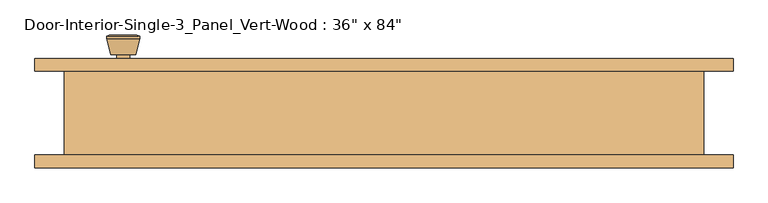
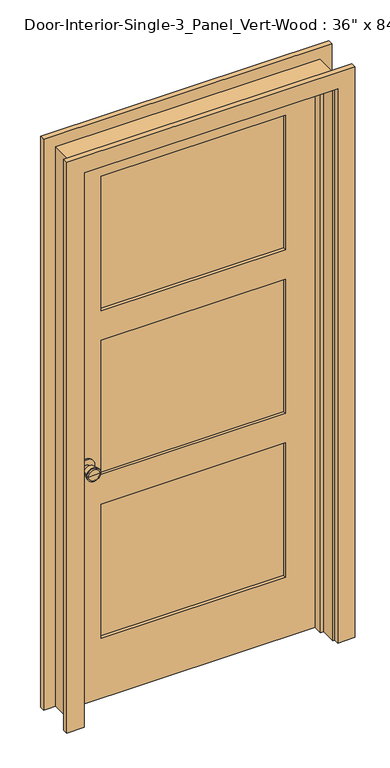
"""IFC4 building model written with IfcOpenShell, lengths in millimetres: door geometry."""

import ifcopenshell
import ifcopenshell.guid

model = None  # the IFC model being written
_history = None  # IfcOwnerHistory: only IFC2X3 demands one
_inside = {}  # id of a spatial element -> (the spatial element, [elements in it])
_under = {}  # id of a project, library or spatial element -> (it, [spatial elements below it])
_declared = {}  # id of a project -> (the project, [libraries it declares])
_typed = {}  # id of a type object -> (the type object, [elements of that type])
_made_of = {}  # id of a material, layer set ... -> (it, [elements and type objects made of it])


def new_model(schema):
    """Start an empty IFC model of exactly this schema.

    Asked for "IFC4X3", IfcOpenShell would pick the latest addendum, in which some entities
    have other attributes; the version numbers below select the first issue.
    IFC2X3 requires an IfcOwnerHistory on every rooted entity: one is made here for all.
    """
    global model, _history
    if schema == "IFC4X3":
        model = ifcopenshell.file(schema_version=(4, 3, 0, 0))
    else:
        model = ifcopenshell.file(schema=schema)
    _inside.clear()
    _under.clear()
    _declared.clear()
    _typed.clear()
    _made_of.clear()
    _history = None
    if model.schema == "IFC2X3":
        org = make("IfcOrganization", Name="unknown")
        user = make(
            "IfcPersonAndOrganization",
            ThePerson=make("IfcPerson", FamilyName="unknown"),
            TheOrganization=org,
        )
        app = make(
            "IfcApplication",
            ApplicationDeveloper=org,
            Version="unknown",
            ApplicationFullName="unknown",
            ApplicationIdentifier="unknown",
        )
        _history = make(
            "IfcOwnerHistory",
            OwningUser=user,
            OwningApplication=app,
            ChangeAction="ADDED",
            CreationDate=0,
        )
    return model


def make(cls, **values):
    """One entity of the class cls with the attributes given. An attribute that is None is left unset."""
    return model.create_entity(
        cls, **{name: value for name, value in values.items() if value is not None}
    )


def rooted(cls, **values):
    """An entity with a GlobalId (a new one), such as an element, a storey or a relation."""
    return make(cls, GlobalId=ifcopenshell.guid.new(), OwnerHistory=_history, **values)


def si_unit(unit_type, name, prefix=None):
    """IfcSIUnit, for example si_unit("LENGTHUNIT", "METRE", prefix="MILLI")."""
    return make("IfcSIUnit", UnitType=unit_type, Prefix=prefix, Name=name)


def assignment(units):
    """IfcUnitAssignment: the units of a project."""
    return None if units is None else make("IfcUnitAssignment", Units=units)


def point(xyz):
    """IfcCartesianPoint."""
    return None if xyz is None else make("IfcCartesianPoint", Coordinates=xyz)


def direction(xyz):
    """IfcDirection."""
    return None if xyz is None else make("IfcDirection", DirectionRatios=xyz)


def frame(location, z_axis=None, x_axis=None):
    """IfcAxis2Placement3D, a coordinate frame: its origin and axes. An axis left out is left unset."""
    return make(
        "IfcAxis2Placement3D",
        Location=point(location),
        Axis=direction(z_axis),
        RefDirection=direction(x_axis),
    )


def frame_2d(location, x_axis=None):
    """IfcAxis2Placement2D, a coordinate frame in the plane: its origin and x axis."""
    return make(
        "IfcAxis2Placement2D", Location=point(location), RefDirection=direction(x_axis)
    )


def origin():
    """The frame at (0, 0, 0) with its axes left unset."""
    return frame((0.0, 0.0, 0.0))


def place(relative_to, where):
    """IfcLocalPlacement: puts the frame where relative to a parent placement (None: the world)."""
    return make(
        "IfcLocalPlacement", PlacementRelTo=relative_to, RelativePlacement=where
    )


def context(
    kind, dimensions, precision=None, world=None, true_north=None, identifier=None
):
    """IfcGeometricRepresentationContext, for example the 3D "Model" context."""
    return make(
        "IfcGeometricRepresentationContext",
        ContextIdentifier=identifier,
        ContextType=kind,
        CoordinateSpaceDimension=dimensions,
        Precision=precision,
        WorldCoordinateSystem=world,
        TrueNorth=true_north,
    )


def project(units=None, contexts=None):
    """IfcProject with its units and contexts."""
    return rooted(
        "IfcProject",
        Name="project",
        RepresentationContexts=contexts,
        UnitsInContext=assignment(units),
    )


def spatial(cls, under=None, at=None, **own):
    """A site, building, storey or space (cls), placed at a placement, below another one or the project."""
    s = rooted(cls, ObjectPlacement=at, **own)
    if under is not None:
        _under.setdefault(under.id(), (under, []))[1].append(s)
    return s


def polyline(points):
    """IfcPolyline through the points."""
    return make("IfcPolyline", Points=[point(p) for p in points])


def circle_curve(where, radius):
    """IfcCircle in the frame where."""
    return make("IfcCircle", Position=where, Radius=radius)


def trimmed(basis, trim1, trim2, sense, master):
    """IfcTrimmedCurve: the piece of a basis curve between two trims."""
    return make(
        "IfcTrimmedCurve",
        BasisCurve=basis,
        Trim1=trim1,
        Trim2=trim2,
        SenseAgreement=sense,
        MasterRepresentation=master,
    )


def segment(curve, same_sense, transition):
    """IfcCompositeCurveSegment."""
    return make(
        "IfcCompositeCurveSegment",
        Transition=transition,
        SameSense=same_sense,
        ParentCurve=curve,
    )


def composite_curve(segments, self_intersect=None):
    """IfcCompositeCurve: segments joined end to end."""
    return make("IfcCompositeCurve", Segments=segments, SelfIntersect=self_intersect)


def outline(outer, holes=None, kind="AREA"):
    """IfcArbitraryClosedProfileDef: a profile drawn as a closed curve; with holes, ...WithVoids."""
    if holes is None:
        return make("IfcArbitraryClosedProfileDef", ProfileType=kind, OuterCurve=outer)
    return make(
        "IfcArbitraryProfileDefWithVoids",
        ProfileType=kind,
        OuterCurve=outer,
        InnerCurves=holes,
    )


def extrude(swept, where, along, depth):
    """IfcExtrudedAreaSolid: the profile swept, set in the frame where, extruded along a direction by depth."""
    return make(
        "IfcExtrudedAreaSolid",
        SweptArea=swept,
        Position=where,
        ExtrudedDirection=direction(along),
        Depth=depth,
    )


def faces_of(points, faces, orient=None, outer=None):
    """IfcFace entities. A face is a list of loops; a loop is a list of indices into points, from 0.

    orient and outer hold one flag for each loop. By default every Orientation is true, the
    first loop of a face is its IfcFaceOuterBound and the others are IfcFaceBound.
    """
    made = []
    for i, loops in enumerate(faces):
        bounds = []
        for j, loop in enumerate(loops):
            is_outer = j == 0 if outer is None else outer[i][j]
            bounds.append(
                make(
                    "IfcFaceOuterBound" if is_outer else "IfcFaceBound",
                    Bound=make("IfcPolyLoop", Polygon=[points[k] for k in loop]),
                    Orientation=True if orient is None else orient[i][j],
                )
            )
        made.append(make("IfcFace", Bounds=bounds))
    return made


def faceted_brep(points, faces, orient=None, outer=None, voids=None):
    """IfcFacetedBrep: a solid bounded by flat faces; with voids (closed shells), ...WithVoids."""
    shared = [point(p) for p in points]
    hull = make("IfcClosedShell", CfsFaces=faces_of(shared, faces, orient, outer))
    if voids is None:
        return make("IfcFacetedBrep", Outer=hull)
    return make(
        "IfcFacetedBrepWithVoids",
        Outer=hull,
        Voids=[
            make(cls, CfsFaces=faces_of(shared, fs, o, b)) for cls, fs, o, b in voids
        ],
    )


def shape(context_of_items, identifier, shape_type, items):
    """IfcShapeRepresentation: the items that make up one representation, for example the "Body"."""
    return make(
        "IfcShapeRepresentation",
        ContextOfItems=context_of_items,
        RepresentationIdentifier=identifier,
        RepresentationType=shape_type,
        Items=items,
    )


def source(mapping_origin, context_of_items, identifier, shape_type, items):
    """IfcRepresentationMap: a shape defined once, which mapped items show again and again."""
    return make(
        "IfcRepresentationMap",
        MappingOrigin=mapping_origin,
        MappedRepresentation=shape(context_of_items, identifier, shape_type, items),
    )


def transform(
    local_origin,
    x_axis=None,
    y_axis=None,
    z_axis=None,
    scale=None,
    scale2=None,
    scale3=None,
    uniform=True,
):
    """IfcCartesianTransformationOperator3D, or its non-uniform kind. x_axis, y_axis, z_axis: its Axis1, 2, 3."""
    if uniform:
        return make(
            "IfcCartesianTransformationOperator3D",
            Axis1=direction(x_axis),
            Axis2=direction(y_axis),
            LocalOrigin=point(local_origin),
            Scale=scale,
            Axis3=direction(z_axis),
        )
    return make(
        "IfcCartesianTransformationOperator3DnonUniform",
        Axis1=direction(x_axis),
        Axis2=direction(y_axis),
        LocalOrigin=point(local_origin),
        Scale=scale,
        Axis3=direction(z_axis),
        Scale2=scale2,
        Scale3=scale3,
    )


def mapped(mapping_source, mapping_target):
    """IfcMappedItem: shows the shape of a source again, moved by a transform."""
    return make(
        "IfcMappedItem", MappingSource=mapping_source, MappingTarget=mapping_target
    )


def made_of(thing, what):
    """Note that an element or type object is made of a material, layer set ...; save() writes the relation."""
    if what is not None:
        _made_of.setdefault(what.id(), (what, []))[1].append(thing)
    return thing


def element(
    cls,
    number,
    at=None,
    inside=None,
    cuts=None,
    type_object=None,
    material=None,
    context=None,
    identifier="Body",
    shape_type=None,
    held_by="IfcProductDefinitionShape",
    body=None,
    shapes=None,
    **own,
):
    """One element of the class cls, such as IfcWall. Its Tag is "e" and its number.

    at: its placement. inside: the storey or other place that contains it. cuts: it is an
    opening in that element (IfcRelVoidsElement). A single representation is given by context,
    identifier, shape_type and body (its items); several are given by shapes. held_by: the class
    of the entity that holds the representations. save() writes the other relations.
    """
    e = rooted(cls, Tag="e%d" % number, ObjectPlacement=at, **own)
    if body is not None:
        shapes = [shape(context, identifier, shape_type, body)]
    if shapes is not None:
        e.Representation = make(held_by, Representations=shapes)
    if inside is not None:
        _inside.setdefault(inside.id(), (inside, []))[1].append(e)
    if cuts is not None:
        rooted(
            "IfcRelVoidsElement", RelatingBuildingElement=cuts, RelatedOpeningElement=e
        )
    if type_object is not None:
        _typed.setdefault(type_object.id(), (type_object, []))[1].append(e)
    return made_of(e, material)


def aggregate(whole, parts):
    """IfcRelAggregates: a whole, such as a stair, and the parts it consists of."""
    return rooted("IfcRelAggregates", RelatingObject=whole, RelatedObjects=parts)


def save(model, path):
    """Write the relations noted so far, then the file.

    IfcRelAggregates (storeys below a building ...), IfcRelContainedInSpatialStructure (elements
    in a storey), IfcRelDefinesByType, IfcRelAssociatesMaterial and IfcRelDeclares: one each for
    every whole, place, type object, material and project.
    """
    for whole, parts in _under.values():
        aggregate(whole, parts)
    for where, things in _inside.values():
        rooted(
            "IfcRelContainedInSpatialStructure",
            RelatedElements=things,
            RelatingStructure=where,
        )
    for kind, things in _typed.values():
        rooted("IfcRelDefinesByType", RelatedObjects=things, RelatingType=kind)
    for what, things in _made_of.values():
        rooted("IfcRelAssociatesMaterial", RelatedObjects=things, RelatingMaterial=what)
    for by, libraries in _declared.values():
        rooted("IfcRelDeclares", RelatingContext=by, RelatedDefinitions=libraries)
    model.write(path)


def plane_surface(at):
    """IfcPlane: the flat surface through the origin of the frame at, square to its z axis."""
    return make("IfcPlane", Position=at)


def cylinder_surface(at, radius):
    """IfcCylindricalSurface: all points at the distance radius from the z axis of the frame at."""
    return make("IfcCylindricalSurface", Position=at, Radius=radius)


def revolved_surface(curve, axis_point, axis_direction):
    """IfcSurfaceOfRevolution: the curve turned about the line through axis_point along axis_direction."""
    return make(
        "IfcSurfaceOfRevolution",
        SweptCurve=make("IfcArbitraryOpenProfileDef", ProfileType="CURVE", Curve=curve),
        AxisPosition=make("IfcAxis1Placement", Location=point(axis_point), Axis=direction(axis_direction)),
    )


def advanced_brep(points, edges, surfaces, faces):
    """IfcAdvancedBrep: a solid bounded by faces that lie on surfaces and meet in shared edges.

    An edge is (start, end): straight between two places in points (the first is 0);
    or (start, end, curve); or (start, end, curve, False) where it runs against its curve.
    A face is (place in surfaces, loops), or (place, loops, False) where it looks against
    its surface's normal. A loop lists edges by number (the first is 1), with a minus sign
    where the edge is run from its end to its start. The first loop is the outer one.
    """
    corners = [point(p) for p in points]
    vertices = [make("IfcVertexPoint", VertexGeometry=c) for c in corners]
    made = []
    for start, end, *more in edges:
        made.append(
            make(
                "IfcEdgeCurve",
                EdgeStart=vertices[start],
                EdgeEnd=vertices[end],
                EdgeGeometry=more[0] if more else make("IfcPolyline", Points=[corners[start], corners[end]]),
                SameSense=more[1] if len(more) > 1 else True,
            )
        )
    hull = []
    for where, loops, *sense in faces:
        bounds = []
        for j, loop in enumerate(loops):
            ring = [make("IfcOrientedEdge", EdgeElement=made[abs(k) - 1], Orientation=k > 0) for k in loop]
            bounds.append(
                make(
                    "IfcFaceOuterBound" if j == 0 else "IfcFaceBound",
                    Bound=make("IfcEdgeLoop", EdgeList=ring),
                    Orientation=True,
                )
            )
        hull.append(make("IfcAdvancedFace", Bounds=bounds, FaceSurface=surfaces[where], SameSense=sense[0] if sense else True))
    return make("IfcAdvancedBrep", Outer=make("IfcClosedShell", CfsFaces=hull))


def door_074fb280(model_context):
    return source(origin(), model_context, "Body", "SolidModel", [
        advanced_brep(
        [(-393.7, 19.4, 914.4), (-383.7, 19.4, 914.4), (-403.7, 19.4, 914.4), (-373.2241324, -29.6, 914.4), (-393.7, -29.6, 914.4), (-414.1758676, -29.6, 914.4), (-368.7, -27.7721319, 914.4), (-418.7, -27.7721319, 914.4), (-368.7, -24.3084537, 914.4), (-418.7, -24.3084537, 914.4), (-375.063764, 0.4, 914.4), (-412.336236, 0.4, 914.4), (-383.7, 0.4, 914.4), (-403.7, 0.4, 914.4)],
        [
            (0, 1),
            (1, 2, circle_curve(frame((-393.7, 19.4, 914.4), z_axis=(0.0, 1.0, 0.0), x_axis=(-1.0, 0.0, 0.0)), 10.0)),
            (2, 0),
            (2, 1, circle_curve(frame((-393.7, 19.4, 914.4), z_axis=(0.0, 1.0, 0.0), x_axis=(-1.0, 0.0, 0.0)), 10.0)),
            (3, 4),
            (4, 5),
            (5, 3, circle_curve(frame((-393.7, -29.6, 914.4), z_axis=(0.0, -1.0, 0.0), x_axis=(-1.0, 0.0, 0.0)), 20.4758676)),
            (3, 5, circle_curve(frame((-393.7, -29.6, 914.4), z_axis=(0.0, -1.0, 0.0), x_axis=(-1.0, 0.0, 0.0)), 20.4758676)),
            (6, 3),
            (5, 7),
            (7, 6, circle_curve(frame((-393.7, -27.7721319, 914.4), z_axis=(0.0, -1.0, 0.0), x_axis=(-1.0, 0.0, 0.0)), 25.0)),
            (6, 7, circle_curve(frame((-393.7, -27.7721319, 914.4), z_axis=(0.0, -1.0, 0.0), x_axis=(-1.0, 0.0, 0.0)), 25.0)),
            (8, 6),
            (7, 9),
            (9, 8, circle_curve(frame((-393.7, -24.3084537, 914.4), z_axis=(0.0, -1.0, 0.0), x_axis=(-1.0, 0.0, 0.0)), 25.0)),
            (8, 9, circle_curve(frame((-393.7, -24.3084537, 914.4), z_axis=(0.0, -1.0, 0.0), x_axis=(-1.0, 0.0, 0.0)), 25.0)),
            (10, 8),
            (9, 11),
            (11, 10, circle_curve(frame((-393.7, 0.4, 914.4), z_axis=(0.0, -1.0, 0.0), x_axis=(-1.0, 0.0, 0.0)), 18.636236)),
            (10, 11, circle_curve(frame((-393.7, 0.4, 914.4), z_axis=(0.0, -1.0, 0.0), x_axis=(-1.0, 0.0, 0.0)), 18.636236)),
            (12, 10),
            (11, 13),
            (13, 12, circle_curve(frame((-393.7, 0.4, 914.4), z_axis=(0.0, -1.0, 0.0), x_axis=(-1.0, 0.0, 0.0)), 10.0)),
            (12, 13, circle_curve(frame((-393.7, 0.4, 914.4), z_axis=(0.0, -1.0, 0.0), x_axis=(-1.0, 0.0, 0.0)), 10.0)),
            (1, 12),
            (13, 2),
        ],
        [
            plane_surface(frame((-393.7, 19.4, 914.4), z_axis=(0.0, 1.0, 0.0), x_axis=(-1.0, 0.0, 0.0))),
            plane_surface(frame((-393.7, -29.6, 914.4), z_axis=(0.0, -1.0, 0.0), x_axis=(-1.0, 0.0, 0.0))),
            revolved_surface(polyline([(-414.1758676, -29.6, 914.4), (-418.7, -27.7721319, 914.4)]), (-393.7, 19.4, 914.4), (0.0, 1.0, 0.0)),
            cylinder_surface(frame((-393.7, 19.4, 914.4), z_axis=(0.0, 1.0, 0.0), x_axis=(-1.0, 0.0, 0.0)), 25.0),
            revolved_surface(polyline([(-418.7, -24.3084537, 914.4), (-412.336236, 0.4, 914.4)]), (-393.7, 19.4, 914.4), (0.0, 1.0, 0.0)),
            plane_surface(frame((-393.7, 0.4, 914.4), z_axis=(0.0, 1.0, 0.0), x_axis=(-1.0, 0.0, 0.0))),
            cylinder_surface(frame((-393.7, 19.4, 914.4), z_axis=(0.0, 1.0, 0.0), x_axis=(-1.0, 0.0, 0.0)), 10.0),
        ],
        [
            (0, [[1, 2, 3]]),
            (0, [[-3, 4, -1]]),
            (1, [[5, 6, 7]]),
            (1, [[-6, -5, 8]]),
            (2, [[9, -7, 10, 11]]),
            (2, [[-10, -8, -9, 12]]),
            (3, [[13, -11, 14, 15]]),
            (3, [[-14, -12, -13, 16]]),
            (4, [[17, -15, 18, 19]]),
            (4, [[-18, -16, -17, 20]]),
            (5, [[21, -19, 22, 23]]),
            (5, [[-22, -20, -21, 24]]),
            (6, [[25, -23, 26, -2]]),
            (6, [[-26, -24, -25, -4]]),
        ],
    ),
        extrude(outline(composite_curve([segment(trimmed(circle_curve(frame_2d((914.4, -393.7)), 30.0), [point((914.4, -423.7))], [point((914.4, -363.7))], False, "CARTESIAN"), True, "CONTINUOUS"), segment(trimmed(circle_curve(frame_2d((914.4, -393.7)), 30.0), [point((914.4, -363.7))], [point((914.4, -423.7))], False, "CARTESIAN"), True, "CONTINUOUS")], self_intersect=False)), frame((0.0, 19.4, 0.0), z_axis=(0.0, 1.0, 0.0), x_axis=(0.0, 0.0, 1.0)), (0.0, 0.0, 1.0), 6.0),
        advanced_brep(
        [(-393.7, 66.325, 914.4), (-403.7, 66.325, 914.4), (-383.7, 66.325, 914.4), (-373.2241324, 115.325, 914.4), (-414.1758676, 115.325, 914.4), (-393.7, 115.325, 914.4), (-368.7, 113.4971319, 914.4), (-418.7, 113.4971319, 914.4), (-368.7, 110.0334537, 914.4), (-418.7, 110.0334537, 914.4), (-375.063764, 85.325, 914.4), (-412.336236, 85.325, 914.4), (-383.7, 85.325, 914.4), (-403.7, 85.325, 914.4)],
        [
            (0, 1),
            (1, 2, circle_curve(frame((-393.7, 66.325, 914.4), z_axis=(0.0, -1.0, 0.0), x_axis=(-1.0, 0.0, 0.0)), 10.0)),
            (2, 0),
            (2, 1, circle_curve(frame((-393.7, 66.325, 914.4), z_axis=(0.0, -1.0, 0.0), x_axis=(-1.0, 0.0, 0.0)), 10.0)),
            (3, 4, circle_curve(frame((-393.7, 115.325, 914.4), z_axis=(0.0, 1.0, 0.0), x_axis=(-1.0, 0.0, 0.0)), 20.4758676)),
            (4, 5),
            (5, 3),
            (4, 3, circle_curve(frame((-393.7, 115.325, 914.4), z_axis=(0.0, 1.0, 0.0), x_axis=(-1.0, 0.0, 0.0)), 20.4758676)),
            (6, 7, circle_curve(frame((-393.7, 113.4971319, 914.4), z_axis=(0.0, 1.0, 0.0), x_axis=(-1.0, 0.0, 0.0)), 25.0)),
            (7, 4),
            (3, 6),
            (7, 6, circle_curve(frame((-393.7, 113.4971319, 914.4), z_axis=(0.0, 1.0, 0.0), x_axis=(-1.0, 0.0, 0.0)), 25.0)),
            (8, 9, circle_curve(frame((-393.7, 110.0334537, 914.4), z_axis=(0.0, 1.0, 0.0), x_axis=(-1.0, 0.0, 0.0)), 25.0)),
            (9, 7),
            (6, 8),
            (9, 8, circle_curve(frame((-393.7, 110.0334537, 914.4), z_axis=(0.0, 1.0, 0.0), x_axis=(-1.0, 0.0, 0.0)), 25.0)),
            (10, 11, circle_curve(frame((-393.7, 85.325, 914.4), z_axis=(0.0, 1.0, 0.0), x_axis=(-1.0, 0.0, 0.0)), 18.636236)),
            (11, 9),
            (8, 10),
            (11, 10, circle_curve(frame((-393.7, 85.325, 914.4), z_axis=(0.0, 1.0, 0.0), x_axis=(-1.0, 0.0, 0.0)), 18.636236)),
            (12, 13, circle_curve(frame((-393.7, 85.325, 914.4), z_axis=(0.0, 1.0, 0.0), x_axis=(-1.0, 0.0, 0.0)), 10.0)),
            (13, 11),
            (10, 12),
            (13, 12, circle_curve(frame((-393.7, 85.325, 914.4), z_axis=(0.0, 1.0, 0.0), x_axis=(-1.0, 0.0, 0.0)), 10.0)),
            (1, 13),
            (12, 2),
        ],
        [
            plane_surface(frame((-393.7, 66.325, 914.4), z_axis=(0.0, -1.0, 0.0), x_axis=(-1.0, 0.0, 0.0))),
            plane_surface(frame((-393.7, 115.325, 914.4), z_axis=(0.0, 1.0, 0.0), x_axis=(-1.0, 0.0, 0.0))),
            revolved_surface(polyline([(-414.1758676, 115.325, 914.4), (-418.7, 113.4971319, 914.4)]), (-393.7, 66.325, 914.4), (0.0, -1.0, 0.0)),
            cylinder_surface(frame((-393.7, 66.325, 914.4), z_axis=(0.0, -1.0, 0.0), x_axis=(-1.0, 0.0, 0.0)), 25.0),
            revolved_surface(polyline([(-418.7, 110.0334537, 914.4), (-412.336236, 85.325, 914.4)]), (-393.7, 66.325, 914.4), (0.0, -1.0, 0.0)),
            plane_surface(frame((-393.7, 85.325, 914.4), z_axis=(0.0, -1.0, 0.0), x_axis=(-1.0, 0.0, 0.0))),
            cylinder_surface(frame((-393.7, 66.325, 914.4), z_axis=(0.0, -1.0, 0.0), x_axis=(-1.0, 0.0, 0.0)), 10.0),
        ],
        [
            (0, [[1, 2, 3]]),
            (0, [[-3, 4, -1]]),
            (1, [[5, 6, 7]]),
            (1, [[8, -7, -6]]),
            (2, [[9, 10, -5, 11]]),
            (2, [[12, -11, -8, -10]]),
            (3, [[13, 14, -9, 15]]),
            (3, [[16, -15, -12, -14]]),
            (4, [[17, 18, -13, 19]]),
            (4, [[20, -19, -16, -18]]),
            (5, [[21, 22, -17, 23]]),
            (5, [[24, -23, -20, -22]]),
            (6, [[-2, 25, -21, 26]]),
            (6, [[-4, -26, -24, -25]]),
        ],
    ),
        extrude(outline(composite_curve([segment(trimmed(circle_curve(frame_2d((914.4, -393.7)), 30.0), [point((914.4, -423.7))], [point((914.4, -363.7))], False, "CARTESIAN"), True, "CONTINUOUS"), segment(trimmed(circle_curve(frame_2d((914.4, -393.7)), 30.0), [point((914.4, -363.7))], [point((914.4, -423.7))], False, "CARTESIAN"), True, "CONTINUOUS")], self_intersect=False)), frame((0.0, 60.325, 0.0), z_axis=(0.0, 1.0, 0.0), x_axis=(0.0, 0.0, 1.0)), (0.0, 0.0, 1.0), 6.0),
        extrude(outline(polyline([(336.55, 37.0416667), (-336.55, 37.0416667), (-336.55, 48.6833333), (336.55, 48.6833333), (336.55, 37.0416667)])), frame((0.0, 0.0, 1496.4833333), z_axis=(0.0, 0.0, 1.0), x_axis=(1.0, 0.0, 0.0)), (0.0, 0.0, 1.0), 518.0541667),
        extrude(outline(polyline([(336.55, 37.0416667), (-336.55, 37.0416667), (-336.55, 48.6833333), (336.55, 48.6833333), (336.55, 37.0416667)])), frame((0.0, 0.0, 231.775), z_axis=(0.0, 0.0, 1.0), x_axis=(1.0, 0.0, 0.0)), (0.0, 0.0, 1.0), 518.0541667),
        extrude(outline(polyline([(336.55, 37.0416667), (-336.55, 37.0416667), (-336.55, 48.6833333), (336.55, 48.6833333), (336.55, 37.0416667)])), frame((0.0, 0.0, 864.1291667), z_axis=(0.0, 0.0, 1.0), x_axis=(1.0, 0.0, 0.0)), (0.0, 0.0, 1.0), 518.0541667),
        extrude(outline(polyline([(2133.6, -457.2), (0.0, -457.2), (0.0, 457.2), (2133.6, 457.2), (2133.6, -457.2)]), holes=[polyline([(2014.5375, -336.55), (2014.5375, 336.55), (1496.4833333, 336.55), (1496.4833333, -336.55), (2014.5375, -336.55)]), polyline([(749.8291667, -336.55), (749.8291667, 336.55), (231.775, 336.55), (231.775, -336.55), (749.8291667, -336.55)]), polyline([(1382.1833333, -336.55), (1382.1833333, 336.55), (864.1291667, 336.55), (864.1291667, -336.55), (1382.1833333, -336.55)])]), frame((0.0, 25.4, 0.0), z_axis=(0.0, 1.0, 0.0), x_axis=(0.0, 0.0, 1.0)), (0.0, 0.0, 1.0), 34.925),
        faceted_brep([(482.6, 60.325, 0.0), (482.6, -66.675, 0.0), (457.2, -66.675, 0.0), (457.2, -9.525, 0.0), (444.5, -9.525, 0.0), (444.5, 25.4, 0.0), (457.2, 25.4, 0.0), (457.2, 60.325, 0.0), (482.6, 60.325, 2159.0), (482.6, -66.675, 2159.0), (-482.6, -66.675, 2159.0), (-482.6, -66.675, 0.0), (-457.2, -66.675, 0.0), (-457.2, -66.675, 2133.6), (457.2, -66.675, 2133.6), (457.2, -9.525, 2133.6), (-457.2, -9.525, 2133.6), (-457.2, -9.525, 0.0), (-444.5, -9.525, 0.0), (-444.5, -9.525, 2120.9), (444.5, -9.525, 2120.9), (444.5, 25.4, 2120.9), (-444.5, 25.4, 2120.9), (-444.5, 25.4, 0.0), (-457.2, 25.4, 0.0), (-457.2, 25.4, 2133.6), (457.2, 25.4, 2133.6), (457.2, 60.325, 2133.6), (-457.2, 60.325, 2133.6), (-457.2, 60.325, 0.0), (-482.6, 60.325, 0.0), (-482.6, 60.325, 2159.0)], [[[0, 1, 2, 3, 4, 5, 6, 7]], [[1, 0, 8, 9]], [[2, 1, 9, 10, 11, 12, 13, 14]], [[3, 2, 14, 15]], [[4, 3, 15, 16, 17, 18, 19, 20]], [[5, 4, 20, 21]], [[6, 5, 21, 22, 23, 24, 25, 26]], [[7, 6, 26, 27]], [[0, 7, 27, 28, 29, 30, 31, 8]], [[9, 8, 31, 10]], [[15, 14, 13, 16]], [[21, 20, 19, 22]], [[27, 26, 25, 28]], [[30, 29, 24, 23, 18, 17, 12, 11]], [[10, 31, 30, 11]], [[16, 13, 12, 17]], [[22, 19, 18, 23]], [[28, 25, 24, 29]]]),
        extrude(outline(polyline([(0.0, 463.55), (0.0, 527.05), (2203.45, 527.05), (2203.45, -527.05), (0.0, -527.05), (0.0, -463.55), (2139.95, -463.55), (2139.95, 463.55), (0.0, 463.55)])), frame((0.0, -85.725, 0.0), z_axis=(0.0, 1.0, 0.0), x_axis=(0.0, 0.0, 1.0)), (0.0, 0.0, 1.0), 19.05),
        extrude(outline(polyline([(0.0, 463.55), (0.0, 527.05), (2203.45, 527.05), (2203.45, -527.05), (0.0, -527.05), (0.0, -463.55), (2139.95, -463.55), (2139.95, 463.55), (0.0, 463.55)])), frame((0.0, 60.325, 0.0), z_axis=(0.0, 1.0, 0.0), x_axis=(0.0, 0.0, 1.0)), (0.0, 0.0, 1.0), 19.05),
    ])


if __name__ == "__main__":
    model = new_model("IFC4")
    model_context = context("Model", 3, world=origin())
    ifc_project = project(units=[si_unit("LENGTHUNIT", "METRE", prefix="MILLI")], contexts=[model_context])
    site = spatial("IfcSite", under=ifc_project)
    building = spatial("IfcBuilding", under=site)
    placement = place(None, origin())
    door_shape = door_074fb280(model_context)
    element("IfcDoor", 1, ObjectType="Door-Interior-Single-3_Panel_Vert-Wood : 36\" x 84\"", at=placement, inside=building, context=model_context, shape_type="MappedRepresentation", body=[
        mapped(door_shape, transform((0.0, 0.0, 0.0), x_axis=(1.0, 0.0, 0.0), y_axis=(0.0, 1.0, 0.0), z_axis=(0.0, 0.0, 1.0))),
    ])
    save(model, "model.ifc")

# Revit data of these elements
# Project information
#   Project Issue Date = "Issue Date"
#   Project Status = "Project Status"
#   Client Name = "Owner"
#   Project Address = "Enter address here"
#   Project Name = "Project Name"
#   Project Number = "Project Number"
# Type "Door-Interior-Single-3_Panel_Vert-Wood : 36\" x 84\""
#   Type Mark = "10"
#   Assembly Code = "C1020300"
#   Analytic Construction = "Wooden"
#   Top Rail = 0' - 4 11/16"
#   Thickness = 0' - 1 3/8"
#   Thermal Resistance (R) = 2.5876 (h·ft²·°F)/BTU
#   Swing Angle [instance default] = 90.00°
#   Stiles = 0' - 4 3/4"
#   Rough Width = 3' - 2"
#   Rough Height = 7' - 1"
#   Intermediate Rail = 0' - 4 1/2"
#   Height = 7' - 0"
#   Width = 3' - 0"
#   Heat Transfer Coefficient (U) = 0.3865 BTU/(h·ft²·°F)
#   Bottom Rail = 0' - 9 1/8"
#   Trim Material = Cherry
#   Panel Material = Cherry
#   Frame Material = Cherry
#   Door Handle Material = Aluminum
#   Visual Light Transmittance = 0
#   Solar Heat Gain Coefficient = 0
#   Wall Closure = (empty or 0)
#   Function = (empty or 0)
# Element 1 (IfcDoor, "Door-Interior-Single-3_Panel_Vert-Wood : 36\" x 84\"")
#   Materials on its faces: "Cherry", "Aluminum"
# Materials
#   "Cherry": class "Wood", colour RGB 226 177 128, transparency 0, Description = "Prunus Serotina", Cost = 0
#   "Aluminum": class "Metal", colour RGB 247 247 247, transparency 0, Description = "Aluminum 6061", Cost = 0
